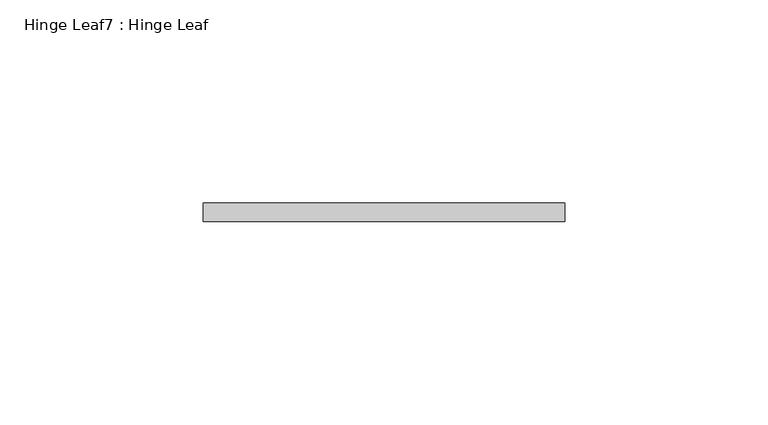
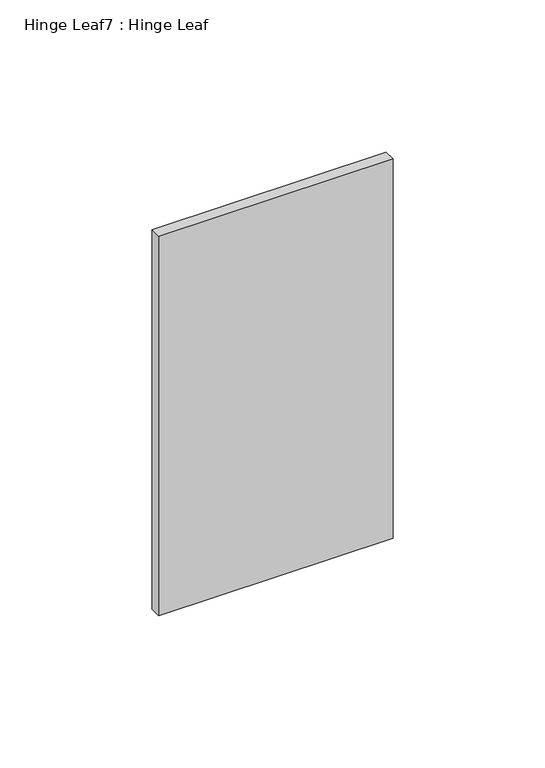
"""IFC4 building model written with IfcOpenShell, lengths in millimetres: proxy geometry, Hinge Leaf7 : Hinge Leaf."""

import ifcopenshell
import ifcopenshell.guid

model = None  # the IFC model being written
_history = None  # IfcOwnerHistory: only IFC2X3 demands one
_inside = {}  # id of a spatial element -> (the spatial element, [elements in it])
_under = {}  # id of a project, library or spatial element -> (it, [spatial elements below it])
_declared = {}  # id of a project -> (the project, [libraries it declares])
_typed = {}  # id of a type object -> (the type object, [elements of that type])
_made_of = {}  # id of a material, layer set ... -> (it, [elements and type objects made of it])


def new_model(schema):
    """Start an empty IFC model of exactly this schema.

    Asked for "IFC4X3", IfcOpenShell would pick the latest addendum, in which some entities
    have other attributes; the version numbers below select the first issue.
    IFC2X3 requires an IfcOwnerHistory on every rooted entity: one is made here for all.
    """
    global model, _history
    if schema == "IFC4X3":
        model = ifcopenshell.file(schema_version=(4, 3, 0, 0))
    else:
        model = ifcopenshell.file(schema=schema)
    _inside.clear()
    _under.clear()
    _declared.clear()
    _typed.clear()
    _made_of.clear()
    _history = None
    if model.schema == "IFC2X3":
        org = make("IfcOrganization", Name="unknown")
        user = make(
            "IfcPersonAndOrganization",
            ThePerson=make("IfcPerson", FamilyName="unknown"),
            TheOrganization=org,
        )
        app = make(
            "IfcApplication",
            ApplicationDeveloper=org,
            Version="unknown",
            ApplicationFullName="unknown",
            ApplicationIdentifier="unknown",
        )
        _history = make(
            "IfcOwnerHistory",
            OwningUser=user,
            OwningApplication=app,
            ChangeAction="ADDED",
            CreationDate=0,
        )
    return model


def make(cls, **values):
    """One entity of the class cls with the attributes given. An attribute that is None is left unset."""
    return model.create_entity(
        cls, **{name: value for name, value in values.items() if value is not None}
    )


def rooted(cls, **values):
    """An entity with a GlobalId (a new one), such as an element, a storey or a relation."""
    return make(cls, GlobalId=ifcopenshell.guid.new(), OwnerHistory=_history, **values)


def si_unit(unit_type, name, prefix=None):
    """IfcSIUnit, for example si_unit("LENGTHUNIT", "METRE", prefix="MILLI")."""
    return make("IfcSIUnit", UnitType=unit_type, Prefix=prefix, Name=name)


def assignment(units):
    """IfcUnitAssignment: the units of a project."""
    return None if units is None else make("IfcUnitAssignment", Units=units)


def point(xyz):
    """IfcCartesianPoint."""
    return None if xyz is None else make("IfcCartesianPoint", Coordinates=xyz)


def direction(xyz):
    """IfcDirection."""
    return None if xyz is None else make("IfcDirection", DirectionRatios=xyz)


def frame(location, z_axis=None, x_axis=None):
    """IfcAxis2Placement3D, a coordinate frame: its origin and axes. An axis left out is left unset."""
    return make(
        "IfcAxis2Placement3D",
        Location=point(location),
        Axis=direction(z_axis),
        RefDirection=direction(x_axis),
    )


def origin():
    """The frame at (0, 0, 0) with its axes left unset."""
    return frame((0.0, 0.0, 0.0))


def place(relative_to, where):
    """IfcLocalPlacement: puts the frame where relative to a parent placement (None: the world)."""
    return make(
        "IfcLocalPlacement", PlacementRelTo=relative_to, RelativePlacement=where
    )


def context(
    kind, dimensions, precision=None, world=None, true_north=None, identifier=None
):
    """IfcGeometricRepresentationContext, for example the 3D "Model" context."""
    return make(
        "IfcGeometricRepresentationContext",
        ContextIdentifier=identifier,
        ContextType=kind,
        CoordinateSpaceDimension=dimensions,
        Precision=precision,
        WorldCoordinateSystem=world,
        TrueNorth=true_north,
    )


def project(units=None, contexts=None):
    """IfcProject with its units and contexts."""
    return rooted(
        "IfcProject",
        Name="project",
        RepresentationContexts=contexts,
        UnitsInContext=assignment(units),
    )


def spatial(cls, under=None, at=None, **own):
    """A site, building, storey or space (cls), placed at a placement, below another one or the project."""
    s = rooted(cls, ObjectPlacement=at, **own)
    if under is not None:
        _under.setdefault(under.id(), (under, []))[1].append(s)
    return s


def polyline(points):
    """IfcPolyline through the points."""
    return make("IfcPolyline", Points=[point(p) for p in points])


def outline(outer, holes=None, kind="AREA"):
    """IfcArbitraryClosedProfileDef: a profile drawn as a closed curve; with holes, ...WithVoids."""
    if holes is None:
        return make("IfcArbitraryClosedProfileDef", ProfileType=kind, OuterCurve=outer)
    return make(
        "IfcArbitraryProfileDefWithVoids",
        ProfileType=kind,
        OuterCurve=outer,
        InnerCurves=holes,
    )


def extrude(swept, where, along, depth):
    """IfcExtrudedAreaSolid: the profile swept, set in the frame where, extruded along a direction by depth."""
    return make(
        "IfcExtrudedAreaSolid",
        SweptArea=swept,
        Position=where,
        ExtrudedDirection=direction(along),
        Depth=depth,
    )


def shape(context_of_items, identifier, shape_type, items):
    """IfcShapeRepresentation: the items that make up one representation, for example the "Body"."""
    return make(
        "IfcShapeRepresentation",
        ContextOfItems=context_of_items,
        RepresentationIdentifier=identifier,
        RepresentationType=shape_type,
        Items=items,
    )


def source(mapping_origin, context_of_items, identifier, shape_type, items):
    """IfcRepresentationMap: a shape defined once, which mapped items show again and again."""
    return make(
        "IfcRepresentationMap",
        MappingOrigin=mapping_origin,
        MappedRepresentation=shape(context_of_items, identifier, shape_type, items),
    )


def transform(
    local_origin,
    x_axis=None,
    y_axis=None,
    z_axis=None,
    scale=None,
    scale2=None,
    scale3=None,
    uniform=True,
):
    """IfcCartesianTransformationOperator3D, or its non-uniform kind. x_axis, y_axis, z_axis: its Axis1, 2, 3."""
    if uniform:
        return make(
            "IfcCartesianTransformationOperator3D",
            Axis1=direction(x_axis),
            Axis2=direction(y_axis),
            LocalOrigin=point(local_origin),
            Scale=scale,
            Axis3=direction(z_axis),
        )
    return make(
        "IfcCartesianTransformationOperator3DnonUniform",
        Axis1=direction(x_axis),
        Axis2=direction(y_axis),
        LocalOrigin=point(local_origin),
        Scale=scale,
        Axis3=direction(z_axis),
        Scale2=scale2,
        Scale3=scale3,
    )


def mapped(mapping_source, mapping_target):
    """IfcMappedItem: shows the shape of a source again, moved by a transform."""
    return make(
        "IfcMappedItem", MappingSource=mapping_source, MappingTarget=mapping_target
    )


def made_of(thing, what):
    """Note that an element or type object is made of a material, layer set ...; save() writes the relation."""
    if what is not None:
        _made_of.setdefault(what.id(), (what, []))[1].append(thing)
    return thing


def element(
    cls,
    number,
    at=None,
    inside=None,
    cuts=None,
    type_object=None,
    material=None,
    context=None,
    identifier="Body",
    shape_type=None,
    held_by="IfcProductDefinitionShape",
    body=None,
    shapes=None,
    **own,
):
    """One element of the class cls, such as IfcWall. Its Tag is "e" and its number.

    at: its placement. inside: the storey or other place that contains it. cuts: it is an
    opening in that element (IfcRelVoidsElement). A single representation is given by context,
    identifier, shape_type and body (its items); several are given by shapes. held_by: the class
    of the entity that holds the representations. save() writes the other relations.
    """
    e = rooted(cls, Tag="e%d" % number, ObjectPlacement=at, **own)
    if body is not None:
        shapes = [shape(context, identifier, shape_type, body)]
    if shapes is not None:
        e.Representation = make(held_by, Representations=shapes)
    if inside is not None:
        _inside.setdefault(inside.id(), (inside, []))[1].append(e)
    if cuts is not None:
        rooted(
            "IfcRelVoidsElement", RelatingBuildingElement=cuts, RelatedOpeningElement=e
        )
    if type_object is not None:
        _typed.setdefault(type_object.id(), (type_object, []))[1].append(e)
    return made_of(e, material)


def aggregate(whole, parts):
    """IfcRelAggregates: a whole, such as a stair, and the parts it consists of."""
    return rooted("IfcRelAggregates", RelatingObject=whole, RelatedObjects=parts)


def save(model, path):
    """Write the relations noted so far, then the file.

    IfcRelAggregates (storeys below a building ...), IfcRelContainedInSpatialStructure (elements
    in a storey), IfcRelDefinesByType, IfcRelAssociatesMaterial and IfcRelDeclares: one each for
    every whole, place, type object, material and project.
    """
    for whole, parts in _under.values():
        aggregate(whole, parts)
    for where, things in _inside.values():
        rooted(
            "IfcRelContainedInSpatialStructure",
            RelatedElements=things,
            RelatingStructure=where,
        )
    for kind, things in _typed.values():
        rooted("IfcRelDefinesByType", RelatedObjects=things, RelatingType=kind)
    for what, things in _made_of.values():
        rooted("IfcRelAssociatesMaterial", RelatedObjects=things, RelatingMaterial=what)
    for by, libraries in _declared.values():
        rooted("IfcRelDeclares", RelatingContext=by, RelatedDefinitions=libraries)
    model.write(path)


def hinge_leaf7_hinge_leaf_106c3047(model_context):
    return source(origin(), model_context, "Body", "SweptSolid", [
        extrude(outline(polyline([(587327.7934739, -533988.7163841), (587327.7934739, -533984.1443841), (587416.6934739, -533984.1443841), (587416.6934739, -533988.7163841), (587327.7934739, -533988.7163841)])), frame((0.0, 0.0, 311.15), z_axis=(0.0, 0.0, 1.0), x_axis=(1.0, 0.0, 0.0)), (0.0, 0.0, 1.0), 152.4),
    ])


if __name__ == "__main__":
    model = new_model("IFC4")
    model_context = context("Model", 3, world=origin())
    ifc_project = project(units=[si_unit("LENGTHUNIT", "METRE", prefix="MILLI")], contexts=[model_context])
    site = spatial("IfcSite", under=ifc_project)
    building = spatial("IfcBuilding", under=site)
    placement = place(None, origin())
    hinge_leaf7_hinge_leaf_shape = hinge_leaf7_hinge_leaf_106c3047(model_context)
    element("IfcBuildingElementProxy", 1, Name="Hinge Leaf7 : Hinge Leaf", ObjectType="Hinge Leaf7 : Hinge Leaf", at=placement, inside=building, context=model_context, shape_type="MappedRepresentation", body=[
        mapped(hinge_leaf7_hinge_leaf_shape, transform((0.0, 0.0, 0.0), x_axis=(1.0, 0.0, 0.0), y_axis=(0.0, 1.0, 0.0), z_axis=(0.0, 0.0, 1.0))),
    ])
    save(model, "model.ifc")

# Revit data of these elements
# Element 1 (IfcBuildingElementProxy, "Hinge Leaf7 : Hinge Leaf")
#   Materials on its faces: "6\"X6\" WELD-ON STL BUTT HINGE"
# Materials
#   "6\"X6\" WELD-ON STL BUTT HINGE": class "Metal", colour RGB 189 187 185, transparency 0, Description = "Carbon steel", Cost = 0
